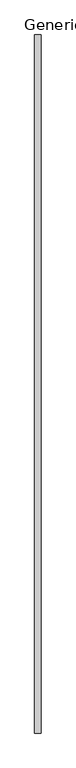
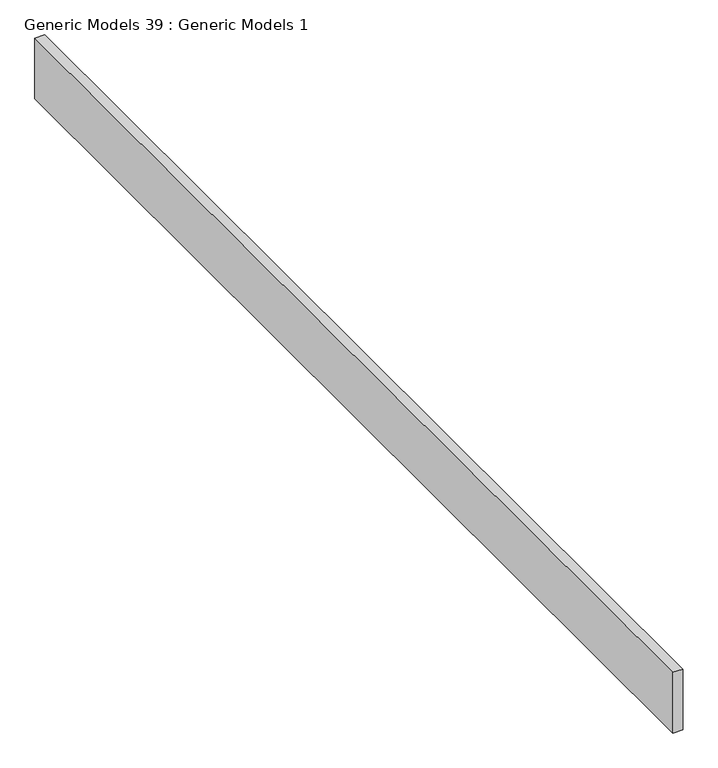
"""IFC4 building model written with IfcOpenShell, lengths in millimetres: proxy geometry, Generic Models 39 : Generic Models 1."""

from ifc_helpers import new_model, si_unit, frame, origin, place, context, project, spatial, polyline, outline, extrude, source, transform, mapped, element, save


def generic_models_39_generic_models_1_38d10ff0(model_context):
    return source(origin(), model_context, "Body", "SweptSolid", [
        extrude(outline(polyline([(-9430.3388857, 11981.8769662), (-9385.8888857, 11981.8769662), (-9385.8888857, 7054.2769662), (-9430.3388857, 7054.2769662), (-9430.3388857, 11981.8769662)])), frame((0.0, 0.0, 126333.4112561), z_axis=(0.0, 0.0, 1.0), x_axis=(1.0, 0.0, 0.0)), (0.0, 0.0, 1.0), 285.75),
    ])


if __name__ == "__main__":
    model = new_model("IFC4")
    model_context = context("Model", 3, world=origin())
    ifc_project = project(units=[si_unit("LENGTHUNIT", "METRE", prefix="MILLI")], contexts=[model_context])
    site = spatial("IfcSite", under=ifc_project)
    building = spatial("IfcBuilding", under=site)
    placement = place(None, origin())
    generic_models_39_generic_models_1_shape = generic_models_39_generic_models_1_38d10ff0(model_context)
    element("IfcBuildingElementProxy", 1, Name="Generic Models 39 : Generic Models 1", ObjectType="Generic Models 39 : Generic Models 1", at=placement, inside=building, context=model_context, shape_type="MappedRepresentation", body=[
        mapped(generic_models_39_generic_models_1_shape, transform((0.0, 0.0, 0.0), x_axis=(1.0, 0.0, 0.0), y_axis=(0.0, 1.0, 0.0), z_axis=(0.0, 0.0, 1.0))),
    ])
    save(model, "model.ifc")

# Revit data of these elements
# Element 1 (IfcBuildingElementProxy, "Generic Models 39 : Generic Models 1")
#   Materials on its faces: "_STRUCTURAL MEMBER (SEE STRUCT. DWGS)"
# Materials
#   "_STRUCTURAL MEMBER (SEE STRUCT. DWGS)": class "Generic", colour RGB 209 182 141, transparency 0, Cost = 0
